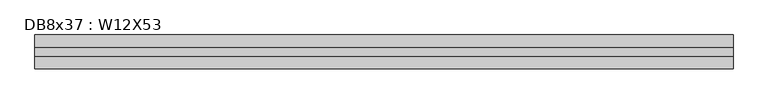
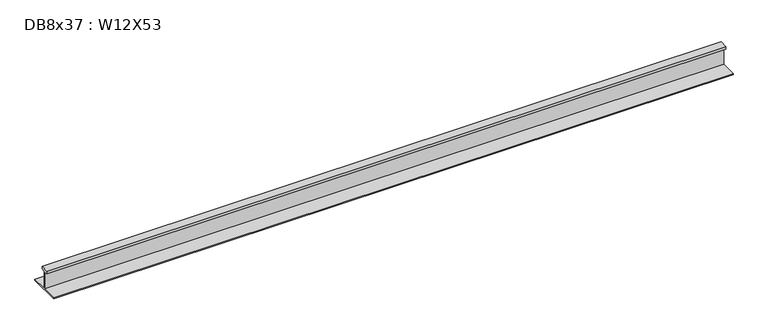
"""IFC4 building model written with IfcOpenShell, lengths in millimetres: beam geometry, DB8x37 : W12X53."""

import ifcopenshell
import ifcopenshell.guid

model = None  # the IFC model being written
_history = None  # IfcOwnerHistory: only IFC2X3 demands one
_inside = {}  # id of a spatial element -> (the spatial element, [elements in it])
_under = {}  # id of a project, library or spatial element -> (it, [spatial elements below it])
_declared = {}  # id of a project -> (the project, [libraries it declares])
_typed = {}  # id of a type object -> (the type object, [elements of that type])
_made_of = {}  # id of a material, layer set ... -> (it, [elements and type objects made of it])


def new_model(schema):
    """Start an empty IFC model of exactly this schema.

    Asked for "IFC4X3", IfcOpenShell would pick the latest addendum, in which some entities
    have other attributes; the version numbers below select the first issue.
    IFC2X3 requires an IfcOwnerHistory on every rooted entity: one is made here for all.
    """
    global model, _history
    if schema == "IFC4X3":
        model = ifcopenshell.file(schema_version=(4, 3, 0, 0))
    else:
        model = ifcopenshell.file(schema=schema)
    _inside.clear()
    _under.clear()
    _declared.clear()
    _typed.clear()
    _made_of.clear()
    _history = None
    if model.schema == "IFC2X3":
        org = make("IfcOrganization", Name="unknown")
        user = make(
            "IfcPersonAndOrganization",
            ThePerson=make("IfcPerson", FamilyName="unknown"),
            TheOrganization=org,
        )
        app = make(
            "IfcApplication",
            ApplicationDeveloper=org,
            Version="unknown",
            ApplicationFullName="unknown",
            ApplicationIdentifier="unknown",
        )
        _history = make(
            "IfcOwnerHistory",
            OwningUser=user,
            OwningApplication=app,
            ChangeAction="ADDED",
            CreationDate=0,
        )
    return model


def make(cls, **values):
    """One entity of the class cls with the attributes given. An attribute that is None is left unset."""
    return model.create_entity(
        cls, **{name: value for name, value in values.items() if value is not None}
    )


def rooted(cls, **values):
    """An entity with a GlobalId (a new one), such as an element, a storey or a relation."""
    return make(cls, GlobalId=ifcopenshell.guid.new(), OwnerHistory=_history, **values)


def si_unit(unit_type, name, prefix=None):
    """IfcSIUnit, for example si_unit("LENGTHUNIT", "METRE", prefix="MILLI")."""
    return make("IfcSIUnit", UnitType=unit_type, Prefix=prefix, Name=name)


def assignment(units):
    """IfcUnitAssignment: the units of a project."""
    return None if units is None else make("IfcUnitAssignment", Units=units)


def point(xyz):
    """IfcCartesianPoint."""
    return None if xyz is None else make("IfcCartesianPoint", Coordinates=xyz)


def direction(xyz):
    """IfcDirection."""
    return None if xyz is None else make("IfcDirection", DirectionRatios=xyz)


def frame(location, z_axis=None, x_axis=None):
    """IfcAxis2Placement3D, a coordinate frame: its origin and axes. An axis left out is left unset."""
    return make(
        "IfcAxis2Placement3D",
        Location=point(location),
        Axis=direction(z_axis),
        RefDirection=direction(x_axis),
    )


def origin():
    """The frame at (0, 0, 0) with its axes left unset."""
    return frame((0.0, 0.0, 0.0))


def place(relative_to, where):
    """IfcLocalPlacement: puts the frame where relative to a parent placement (None: the world)."""
    return make(
        "IfcLocalPlacement", PlacementRelTo=relative_to, RelativePlacement=where
    )


def context(
    kind, dimensions, precision=None, world=None, true_north=None, identifier=None
):
    """IfcGeometricRepresentationContext, for example the 3D "Model" context."""
    return make(
        "IfcGeometricRepresentationContext",
        ContextIdentifier=identifier,
        ContextType=kind,
        CoordinateSpaceDimension=dimensions,
        Precision=precision,
        WorldCoordinateSystem=world,
        TrueNorth=true_north,
    )


def project(units=None, contexts=None):
    """IfcProject with its units and contexts."""
    return rooted(
        "IfcProject",
        Name="project",
        RepresentationContexts=contexts,
        UnitsInContext=assignment(units),
    )


def spatial(cls, under=None, at=None, **own):
    """A site, building, storey or space (cls), placed at a placement, below another one or the project."""
    s = rooted(cls, ObjectPlacement=at, **own)
    if under is not None:
        _under.setdefault(under.id(), (under, []))[1].append(s)
    return s


def polyline(points):
    """IfcPolyline through the points."""
    return make("IfcPolyline", Points=[point(p) for p in points])


def outline(outer, holes=None, kind="AREA"):
    """IfcArbitraryClosedProfileDef: a profile drawn as a closed curve; with holes, ...WithVoids."""
    if holes is None:
        return make("IfcArbitraryClosedProfileDef", ProfileType=kind, OuterCurve=outer)
    return make(
        "IfcArbitraryProfileDefWithVoids",
        ProfileType=kind,
        OuterCurve=outer,
        InnerCurves=holes,
    )


def extrude(swept, where, along, depth):
    """IfcExtrudedAreaSolid: the profile swept, set in the frame where, extruded along a direction by depth."""
    return make(
        "IfcExtrudedAreaSolid",
        SweptArea=swept,
        Position=where,
        ExtrudedDirection=direction(along),
        Depth=depth,
    )


def shape(context_of_items, identifier, shape_type, items):
    """IfcShapeRepresentation: the items that make up one representation, for example the "Body"."""
    return make(
        "IfcShapeRepresentation",
        ContextOfItems=context_of_items,
        RepresentationIdentifier=identifier,
        RepresentationType=shape_type,
        Items=items,
    )


def source(mapping_origin, context_of_items, identifier, shape_type, items):
    """IfcRepresentationMap: a shape defined once, which mapped items show again and again."""
    return make(
        "IfcRepresentationMap",
        MappingOrigin=mapping_origin,
        MappedRepresentation=shape(context_of_items, identifier, shape_type, items),
    )


def transform(
    local_origin,
    x_axis=None,
    y_axis=None,
    z_axis=None,
    scale=None,
    scale2=None,
    scale3=None,
    uniform=True,
):
    """IfcCartesianTransformationOperator3D, or its non-uniform kind. x_axis, y_axis, z_axis: its Axis1, 2, 3."""
    if uniform:
        return make(
            "IfcCartesianTransformationOperator3D",
            Axis1=direction(x_axis),
            Axis2=direction(y_axis),
            LocalOrigin=point(local_origin),
            Scale=scale,
            Axis3=direction(z_axis),
        )
    return make(
        "IfcCartesianTransformationOperator3DnonUniform",
        Axis1=direction(x_axis),
        Axis2=direction(y_axis),
        LocalOrigin=point(local_origin),
        Scale=scale,
        Axis3=direction(z_axis),
        Scale2=scale2,
        Scale3=scale3,
    )


def mapped(mapping_source, mapping_target):
    """IfcMappedItem: shows the shape of a source again, moved by a transform."""
    return make(
        "IfcMappedItem", MappingSource=mapping_source, MappingTarget=mapping_target
    )


def made_of(thing, what):
    """Note that an element or type object is made of a material, layer set ...; save() writes the relation."""
    if what is not None:
        _made_of.setdefault(what.id(), (what, []))[1].append(thing)
    return thing


def element(
    cls,
    number,
    at=None,
    inside=None,
    cuts=None,
    type_object=None,
    material=None,
    context=None,
    identifier="Body",
    shape_type=None,
    held_by="IfcProductDefinitionShape",
    body=None,
    shapes=None,
    **own,
):
    """One element of the class cls, such as IfcWall. Its Tag is "e" and its number.

    at: its placement. inside: the storey or other place that contains it. cuts: it is an
    opening in that element (IfcRelVoidsElement). A single representation is given by context,
    identifier, shape_type and body (its items); several are given by shapes. held_by: the class
    of the entity that holds the representations. save() writes the other relations.
    """
    e = rooted(cls, Tag="e%d" % number, ObjectPlacement=at, **own)
    if body is not None:
        shapes = [shape(context, identifier, shape_type, body)]
    if shapes is not None:
        e.Representation = make(held_by, Representations=shapes)
    if inside is not None:
        _inside.setdefault(inside.id(), (inside, []))[1].append(e)
    if cuts is not None:
        rooted(
            "IfcRelVoidsElement", RelatingBuildingElement=cuts, RelatedOpeningElement=e
        )
    if type_object is not None:
        _typed.setdefault(type_object.id(), (type_object, []))[1].append(e)
    return made_of(e, material)


def aggregate(whole, parts):
    """IfcRelAggregates: a whole, such as a stair, and the parts it consists of."""
    return rooted("IfcRelAggregates", RelatingObject=whole, RelatedObjects=parts)


def save(model, path):
    """Write the relations noted so far, then the file.

    IfcRelAggregates (storeys below a building ...), IfcRelContainedInSpatialStructure (elements
    in a storey), IfcRelDefinesByType, IfcRelAssociatesMaterial and IfcRelDeclares: one each for
    every whole, place, type object, material and project.
    """
    for whole, parts in _under.values():
        aggregate(whole, parts)
    for where, things in _inside.values():
        rooted(
            "IfcRelContainedInSpatialStructure",
            RelatedElements=things,
            RelatingStructure=where,
        )
    for kind, things in _typed.values():
        rooted("IfcRelDefinesByType", RelatedObjects=things, RelatingType=kind)
    for what, things in _made_of.values():
        rooted("IfcRelAssociatesMaterial", RelatedObjects=things, RelatingMaterial=what)
    for by, libraries in _declared.values():
        rooted("IfcRelDeclares", RelatingContext=by, RelatedDefinitions=libraries)
    model.write(path)


def db8x37_w12x53_717e7021(model_context):
    return source(origin(), model_context, "Body", "SweptSolid", [
        extrude(outline(polyline([(38.1, 145.415), (38.1, 120.015), (2.921, 120.015), (2.921, -48.4505), (152.4, -48.4505), (152.4, -58.1025), (-152.4, -58.1025), (-152.4, -48.4505), (-2.921, -48.4505), (-2.921, 120.015), (-38.1, 120.015), (-38.1, 145.415), (38.1, 145.415)])), frame((-3135.63, 0.0, 0.0), z_axis=(1.0, 0.0, 0.0), x_axis=(0.0, 1.0, 0.0)), (0.0, 0.0, 1.0), 6301.359),
    ])


if __name__ == "__main__":
    model = new_model("IFC4")
    model_context = context("Model", 3, world=origin())
    ifc_project = project(units=[si_unit("LENGTHUNIT", "METRE", prefix="MILLI")], contexts=[model_context])
    site = spatial("IfcSite", under=ifc_project)
    building = spatial("IfcBuilding", under=site)
    placement = place(None, origin())
    db8x37_w12x53_shape = db8x37_w12x53_717e7021(model_context)
    element("IfcBeam", 1, ObjectType="DB8x37 : W12X53", at=placement, inside=building, context=model_context, shape_type="MappedRepresentation", body=[
        mapped(db8x37_w12x53_shape, transform((0.0, 0.0, 0.0), x_axis=(1.0, 0.0, 0.0), y_axis=(0.0, 1.0, 0.0), z_axis=(0.0, 0.0, 1.0))),
    ])
    save(model, "model.ifc")

# Revit data of these elements
# Type "DB8x37 : W12X53"
#   Assembly Code = "B10"
#   W = 53
#   Length [instance default] = 5' - 0"
#   bf = 0' - 10"
#   d = 1' - 0.1"
#   k = 0' - 1 3/8"
#   k2 = 0' - 0.8"
#   tf = 0' - 0.575"
#   tw = 0' - 0.345"
#   A = 0.108333 SF
#   Structural Material [instance default] = Steel ASTM A992
# Element 1 (IfcBeam, "DB8x37 : W12X53")
#   Materials on its faces: "Steel ASTM A992"
# Materials
#   "Steel ASTM A992": class "Metal", colour RGB 199 199 199, transparency 0, Description = "Structural steel 50ksi", Cost = 0
